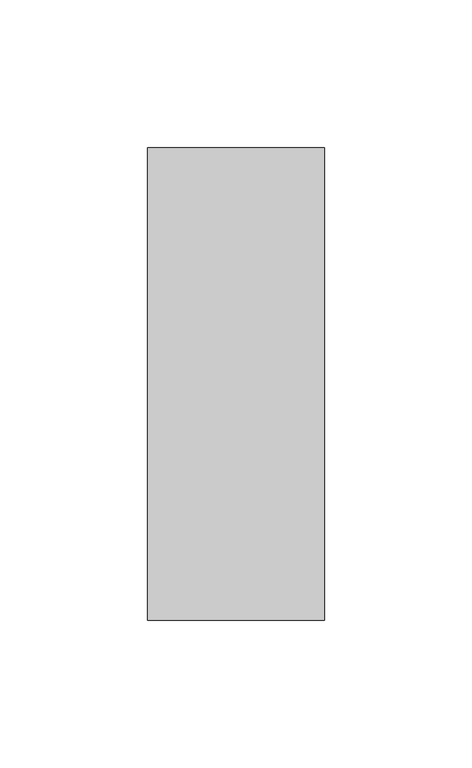
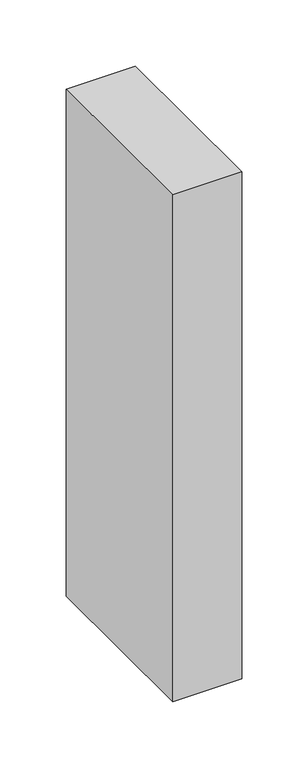
"""IFC4 building model written with IfcOpenShell, lengths in millimetres: column geometry, Madeira de lei-Coluna : Pontalete 6X16cm."""

from ifc_helpers import new_model, si_unit, frame, origin, place, context, project, spatial, polyline, outline, extrude, source, transform, mapped, element, save


def column_7d6827b5(model_context):
    return source(origin(), model_context, "Body", "SweptSolid", [
        extrude(outline(polyline([(30.0, 80.0), (30.0, -80.0), (-30.0, -80.0), (-30.0, 80.0), (30.0, 80.0)])), frame((0.0, 0.0, 4460.0), z_axis=(0.0, 0.0, 1.0), x_axis=(1.0, 0.0, 0.0)), (0.0, 0.0, 1.0), 466.0),
    ])


if __name__ == "__main__":
    model = new_model("IFC4")
    model_context = context("Model", 3, world=origin())
    ifc_project = project(units=[si_unit("LENGTHUNIT", "METRE", prefix="MILLI")], contexts=[model_context])
    site = spatial("IfcSite", under=ifc_project)
    building = spatial("IfcBuilding", under=site)
    placement = place(None, origin())
    column_shape = column_7d6827b5(model_context)
    element("IfcColumn", 1, ObjectType="Madeira de lei-Coluna : Pontalete 6X16cm", at=placement, inside=building, context=model_context, shape_type="MappedRepresentation", body=[
        mapped(column_shape, transform((0.0, 0.0, 0.0), x_axis=(1.0, 0.0, 0.0), y_axis=(0.0, 1.0, 0.0), z_axis=(0.0, 0.0, 1.0))),
    ])
    save(model, "model.ifc")

# Revit data of these elements
# Type "Madeira de lei-Coluna : Pontalete 6X16cm"
#   A = 0.01952 m²
#   b = 0.06 m
#   d = 0.16 m
#   Structural Material [instance default] = none
#   Assembly Code = ""
# Element 1 (IfcColumn, "Madeira de lei-Coluna : Pontalete 6X16cm")
#   Structural Material = .MADEIRAMENTO
#   Materials on its faces: ".MADEIRAMENTO"
# Materials
#   ".MADEIRAMENTO": class ".CC_MADEIRAS", colour RGB 212 179 113, transparency 0, Cost = 0
